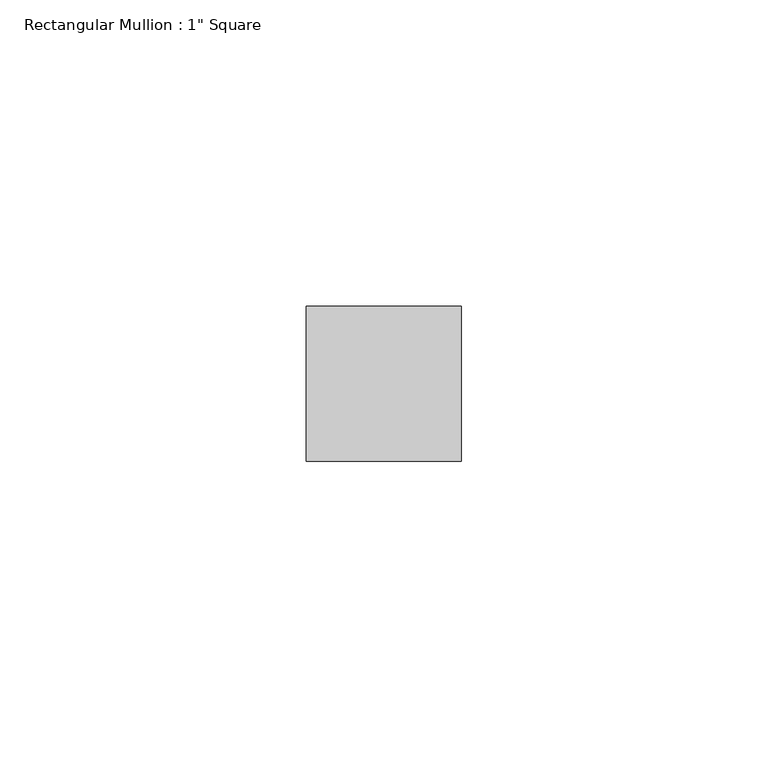
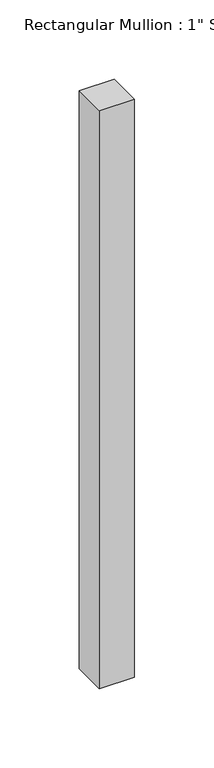
"""IFC4 building model written with IfcOpenShell, lengths in millimetres: member geometry."""

from ifc_helpers import new_model, si_unit, frame, origin, place, context, project, spatial, polyline, outline, extrude, source, transform, mapped, element, save


def member_e8387abb(model_context):
    return source(origin(), model_context, "Body", "SweptSolid", [
        extrude(outline(polyline([(12.7, 12.7), (12.7, -12.7), (-12.7, -12.7), (-12.7, 12.7), (12.7, 12.7)])), frame((0.0, 0.0, -444.5), z_axis=(0.0, 0.0, 1.0), x_axis=(1.0, 0.0, 0.0)), (0.0, 0.0, 1.0), 444.5),
    ])


if __name__ == "__main__":
    model = new_model("IFC4")
    model_context = context("Model", 3, world=origin())
    ifc_project = project(units=[si_unit("LENGTHUNIT", "METRE", prefix="MILLI")], contexts=[model_context])
    site = spatial("IfcSite", under=ifc_project)
    building = spatial("IfcBuilding", under=site)
    placement = place(None, origin())
    member_shape = member_e8387abb(model_context)
    element("IfcMember", 1, ObjectType="Rectangular Mullion : 1\" Square", at=placement, inside=building, context=model_context, shape_type="MappedRepresentation", body=[
        mapped(member_shape, transform((0.0, 0.0, 0.0), x_axis=(1.0, 0.0, 0.0), y_axis=(0.0, 1.0, 0.0), z_axis=(0.0, 0.0, 1.0))),
    ])
    save(model, "model.ifc")

# Revit data of these elements
# Type "Rectangular Mullion : 1\" Square"
#   built-in parameter 1007304 = 0.0833333 (stored number, unit not read)
#   built-in parameter 1007301 = 0.0416667 (stored number, unit not read)
#   built-in parameter 1007300 = 0.0416667 (stored number, unit not read)
# Element 1 (IfcMember, "Rectangular Mullion : 1\" Square")
#   Materials on its faces: "Metal - Aluminum"
# Materials
#   "Metal - Aluminum": class "Metal", colour RGB 247 247 247, transparency 0
